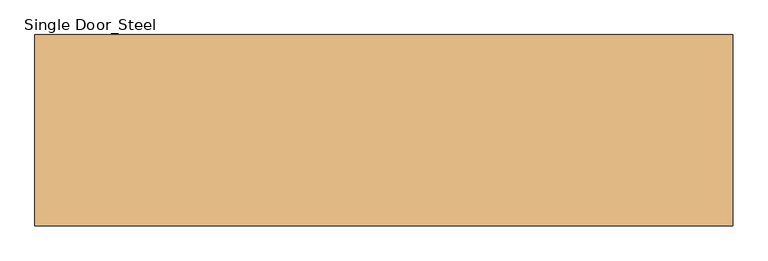
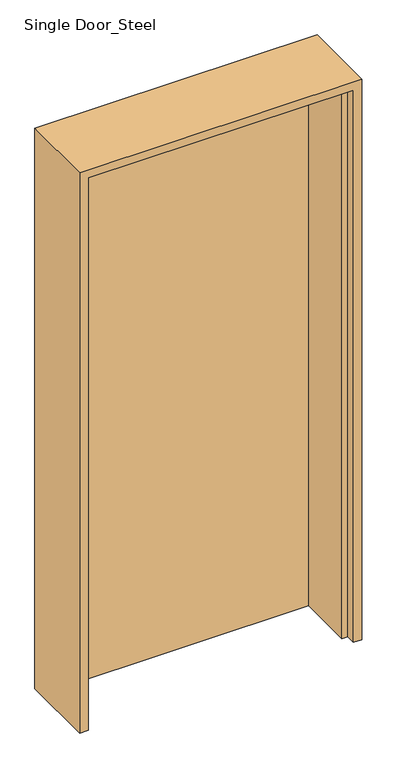
"""IFC4 building model written with IfcOpenShell, lengths in millimetres: door geometry, Single Door_Steel : H_DR_AMD_Single Door_Int_Steel_1000x2100."""

from ifc_helpers import new_model, si_unit, origin, origin_with_axes, place, context, project, spatial, polyline, outline, extrude, faceted_brep, source, transform, mapped, element, save


def single_door_steel_d0b51d4b(model_context):
    return source(origin(), model_context, "Body", "SolidModel", [
        extrude(outline(polyline([(470.0, 137.0), (470.0, 102.0), (-470.0, 102.0), (-470.0, 137.0), (470.0, 137.0)])), origin_with_axes(), (0.0, 0.0, 1.0), 2070.0),
        faceted_brep([(470.0, 137.0, 0.0), (500.0, 137.0, 0.0), (500.0, -137.0, 0.0), (470.0, -137.0, 0.0), (470.0, -102.0, 0.0), (450.0, -102.0, 0.0), (450.0, 102.0, 0.0), (470.0, 102.0, 0.0), (470.0, 137.0, 2070.0), (-470.0, 137.0, 2070.0), (-470.0, 137.0, 0.0), (-500.0, 137.0, 0.0), (-500.0, 137.0, 2100.0), (500.0, 137.0, 2100.0), (500.0, -137.0, 2100.0), (-500.0, -137.0, 2100.0), (-500.0, -137.0, 0.0), (-470.0, -137.0, 0.0), (-470.0, -137.0, 2070.0), (470.0, -137.0, 2070.0), (470.0, -102.0, 2070.0), (-470.0, -102.0, 2070.0), (-470.0, -102.0, 0.0), (-450.0, -102.0, 0.0), (-450.0, -102.0, 2050.0), (450.0, -102.0, 2050.0), (450.0, 102.0, 2050.0), (-450.0, 102.0, 2050.0), (-450.0, 102.0, 0.0), (-470.0, 102.0, 0.0), (-470.0, 102.0, 2070.0), (470.0, 102.0, 2070.0)], [[[0, 1, 2, 3, 4, 5, 6, 7]], [[1, 0, 8, 9, 10, 11, 12, 13]], [[2, 1, 13, 14]], [[3, 2, 14, 15, 16, 17, 18, 19]], [[4, 3, 19, 20]], [[5, 4, 20, 21, 22, 23, 24, 25]], [[6, 5, 25, 26]], [[7, 6, 26, 27, 28, 29, 30, 31]], [[0, 7, 31, 8]], [[9, 30, 29, 10]], [[10, 29, 28, 23, 22, 17, 16, 11]], [[15, 12, 11, 16]], [[21, 18, 17, 22]], [[27, 24, 23, 28]], [[14, 13, 12, 15]], [[20, 19, 18, 21]], [[26, 25, 24, 27]], [[8, 31, 30, 9]]]),
    ])


if __name__ == "__main__":
    model = new_model("IFC4")
    model_context = context("Model", 3, world=origin())
    ifc_project = project(units=[si_unit("LENGTHUNIT", "METRE", prefix="MILLI")], contexts=[model_context])
    site = spatial("IfcSite", under=ifc_project)
    building = spatial("IfcBuilding", under=site)
    placement = place(None, origin())
    single_door_steel_shape = single_door_steel_d0b51d4b(model_context)
    element("IfcDoor", 1, ObjectType="Single Door_Steel : H_DR_AMD_Single Door_Int_Steel_1000x2100", at=placement, inside=building, context=model_context, shape_type="MappedRepresentation", body=[
        mapped(single_door_steel_shape, transform((0.0, 0.0, 0.0), x_axis=(1.0, 0.0, 0.0), y_axis=(0.0, 1.0, 0.0), z_axis=(0.0, 0.0, 1.0))),
    ])
    save(model, "model.ifc")

# Revit data of these elements
# Type "Single Door_Steel : H_DR_AMD_Single Door_Int_Steel_1000x2100"
#   Type Mark = "SD"
#   Analytic Construction = "<None>"
#   프레임 투영 외부. = 0.0250 m
#   프레임 투영 내부. = 0.0250 m
#   프레임 폭 = 0.0750 m
#   Height = 2.1000 m
#   Width = 1.0000 m
#   Define Thermal Properties by = 1
#   문 패널 = SD1 문 패널
#   문 프레임 = A04AR099-00001_Steel Door_Single_FR_N
#   Function = (empty or 0)
#   Wall Closure = (empty or 0)
# Element 1 (IfcDoor, "Single Door_Steel : H_DR_AMD_Single Door_Int_Steel_1000x2100")
#   Materials on its faces: "A04AR099-00001_Steel Door_Single_FR_N", "SD1 문 패널"
# Materials
#   "SD1 문 패널": class "금속", colour RGB 247 247 247, transparency 0, Description = "STEEL DOOR (1000Wx2100H)"
#   "A04AR099-00001_Steel Door_Single_FR_N": class "Metal", colour RGB 247 247 247, transparency 0, Description = "Steel Door w/ Steel Frame", Cost = 0
